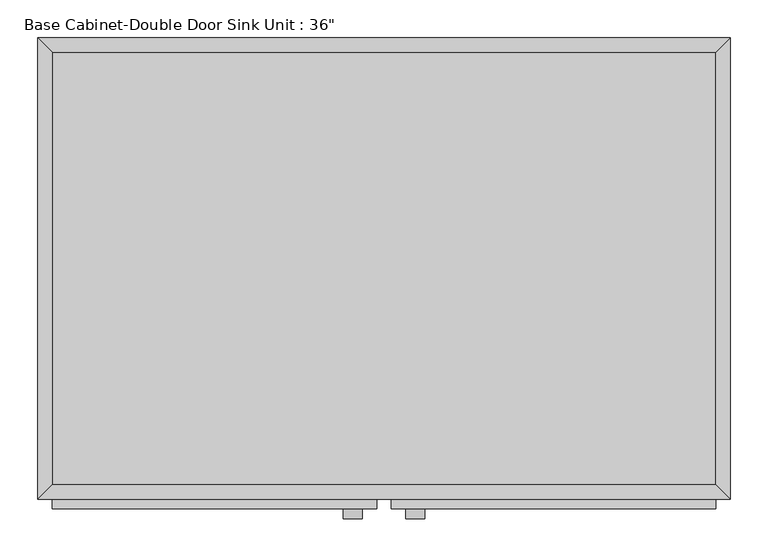
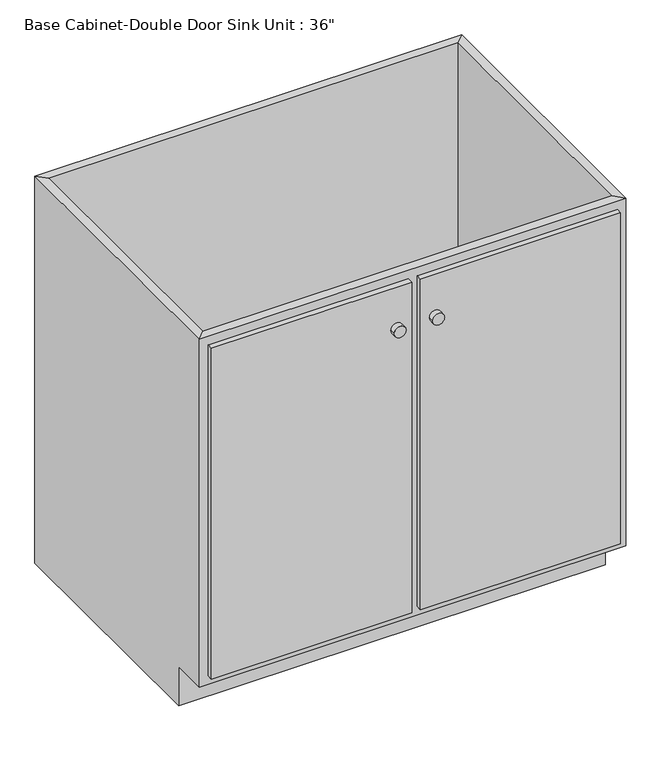
"""IFC4 building model written with IfcOpenShell, lengths in millimetres: furniture geometry."""

from ifc_helpers import new_model, si_unit, point, frame, frame_2d, origin, place, context, project, spatial, polyline, circle_curve, trimmed, segment, composite_curve, outline, extrude, faceted_brep, source, transform, mapped, element, save


def furniture_ee4be6c1(model_context):
    return source(origin(), model_context, "Body", "SolidModel", [
        faceted_brep([(456.8877049, -590.55, 876.3), (456.8877049, -590.55, 88.9), (-419.4122951, -590.55, 88.9), (-419.4122951, -590.55, 876.3), (-438.4622951, -609.6, 876.3), (475.9377049, -609.6, 876.3), (-438.4622951, -609.6, 88.9), (475.9377049, -609.6, 88.9), (-419.4122951, -533.4, 88.9), (-419.4122951, -19.05, 88.9), (-419.4122951, -19.05, 876.3), (-438.4622951, 0.0, 876.3), (-438.4622951, 0.0, 0.0), (-438.4622951, -533.4, 0.0), (-438.4622951, -533.4, 88.9), (456.8877049, -19.05, 88.9), (456.8877049, -19.05, 876.3), (475.9377049, 0.0, 876.3), (475.9377049, 0.0, 0.0), (456.8877049, -533.4, 88.9), (475.9377049, -533.4, 88.9), (475.9377049, -533.4, 0.0)], [[[0, 1, 2, 3]], [[0, 3, 4, 5]], [[5, 4, 6, 7]], [[2, 1, 7, 6]], [[3, 2, 8, 9, 10]], [[4, 3, 10, 11]], [[6, 4, 11, 12, 13, 14]], [[2, 6, 14, 8]], [[10, 9, 15, 16]], [[11, 10, 16, 17]], [[12, 11, 17, 18]], [[1, 0, 16, 15, 19]], [[0, 5, 17, 16]], [[5, 7, 20, 21, 18, 17]], [[7, 1, 19, 20]], [[8, 19, 15, 9]], [[18, 21, 13, 12]], [[13, 21, 20, 19, 8, 14]]]),
        extrude(outline(composite_curve([segment(trimmed(circle_curve(frame_2d((763.1349475, -22.5372951)), 12.7), [point((763.1349475, -35.2372951))], [point((763.1349475, -9.8372951))], False, "CARTESIAN"), True, "CONTINUOUS"), segment(trimmed(circle_curve(frame_2d((763.1349475, -22.5372951)), 12.7), [point((763.1349475, -9.8372951))], [point((763.1349475, -35.2372951))], False, "CARTESIAN"), True, "CONTINUOUS")], self_intersect=False)), frame((0.0, -635.0, 0.0), z_axis=(0.0, 1.0, 0.0), x_axis=(0.0, 0.0, 1.0)), (0.0, 0.0, 1.0), 12.7),
        extrude(outline(composite_curve([segment(trimmed(circle_curve(frame_2d((763.1349475, 60.0127049)), 12.7), [point((763.1349475, 47.3127049))], [point((763.1349475, 72.7127049))], False, "CARTESIAN"), True, "CONTINUOUS"), segment(trimmed(circle_curve(frame_2d((763.1349475, 60.0127049)), 12.7), [point((763.1349475, 72.7127049))], [point((763.1349475, 47.3127049))], False, "CARTESIAN"), True, "CONTINUOUS")], self_intersect=False)), frame((0.0, -635.0, 0.0), z_axis=(0.0, 1.0, 0.0), x_axis=(0.0, 0.0, 1.0)), (0.0, 0.0, 1.0), 12.7),
        extrude(outline(polyline([(456.8877049, -19.05), (456.8877049, -590.55), (-419.4122951, -590.55), (-419.4122951, -19.05), (456.8877049, -19.05)])), frame((0.0, 0.0, 88.9), z_axis=(0.0, 0.0, 1.0), x_axis=(1.0, 0.0, 0.0)), (0.0, 0.0, 1.0), 19.05),
        extrude(outline(polyline([(9.2127049, -622.3), (-419.4122951, -622.3), (-419.4122951, -609.6), (9.2127049, -609.6), (9.2127049, -622.3)])), frame((0.0, 0.0, 107.95), z_axis=(0.0, 0.0, 1.0), x_axis=(1.0, 0.0, 0.0)), (0.0, 0.0, 1.0), 749.3),
        extrude(outline(polyline([(456.8877049, -622.3), (28.2627049, -622.3), (28.2627049, -609.6), (456.8877049, -609.6), (456.8877049, -622.3)])), frame((0.0, 0.0, 107.95), z_axis=(0.0, 0.0, 1.0), x_axis=(1.0, 0.0, 0.0)), (0.0, 0.0, 1.0), 749.3),
    ])


if __name__ == "__main__":
    model = new_model("IFC4")
    model_context = context("Model", 3, world=origin())
    ifc_project = project(units=[si_unit("LENGTHUNIT", "METRE", prefix="MILLI")], contexts=[model_context])
    site = spatial("IfcSite", under=ifc_project)
    building = spatial("IfcBuilding", under=site)
    placement = place(None, origin())
    furniture_shape = furniture_ee4be6c1(model_context)
    element("IfcFurniture", 1, ObjectType="Base Cabinet-Double Door Sink Unit : 36\"", at=placement, inside=building, context=model_context, shape_type="MappedRepresentation", body=[
        mapped(furniture_shape, transform((0.0, 0.0, 0.0), x_axis=(1.0, 0.0, 0.0), y_axis=(0.0, 1.0, 0.0), z_axis=(0.0, 0.0, 1.0))),
    ])
    save(model, "model.ifc")

# Revit data of these elements
# Type "Base Cabinet-Double Door Sink Unit : 36\""
#   Assembly Code = "C1030410"
#   Depth = 2' - 0"
#   Height = 2' - 10 1/2"
#   Toe Depth = 0' - 3"
#   Toe Height = 0' - 3 1/2"
#   Width = 3' - 0"
#   Cabinet Material = Base cabinet 2120100 Aspekt - 83012120100 - White
#   Door/Drawer Material = Base cabinet 2120100 Aspekt - 83012120100 - White
#   Handle Material = Cabinets - Handles
#   Default Elevation = 0
# Element 1 (IfcFurniture, "Base Cabinet-Double Door Sink Unit : 36\"")
#   Materials on its faces: "Base cabinet 2120100 Aspekt - 83012120100 - White", "Cabinets - Handles"
# Materials
#   "Base cabinet 2120100 Aspekt - 83012120100 - White": class "Miscellaneous", colour RGB 255 255 255, transparency 0, Manufacturer = "Marbodal", URL = "http://www.marbodal.se", Cost = 0
#   "Cabinets - Handles": class "Metal", colour RGB 57 57 57, transparency 0
